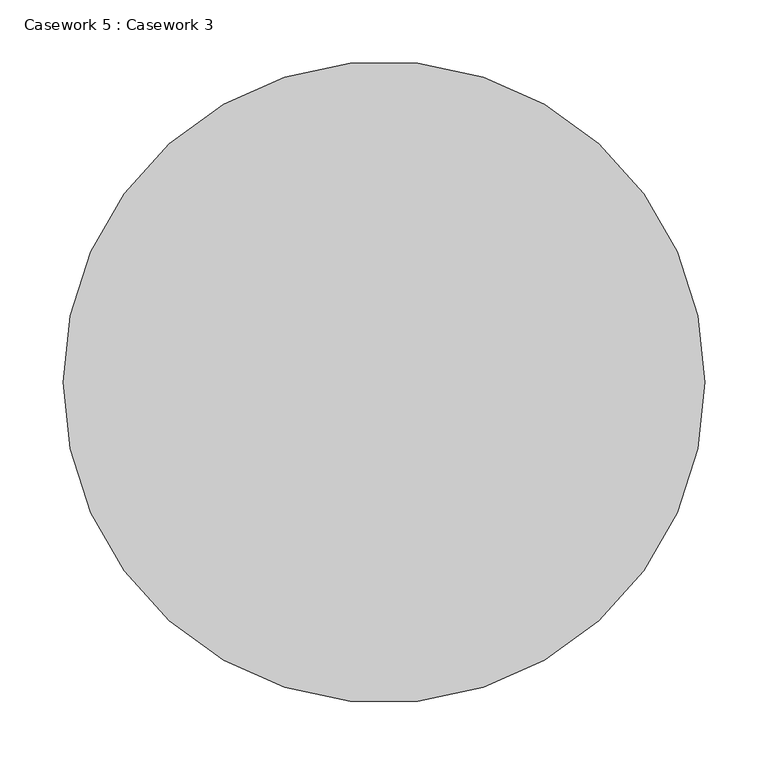
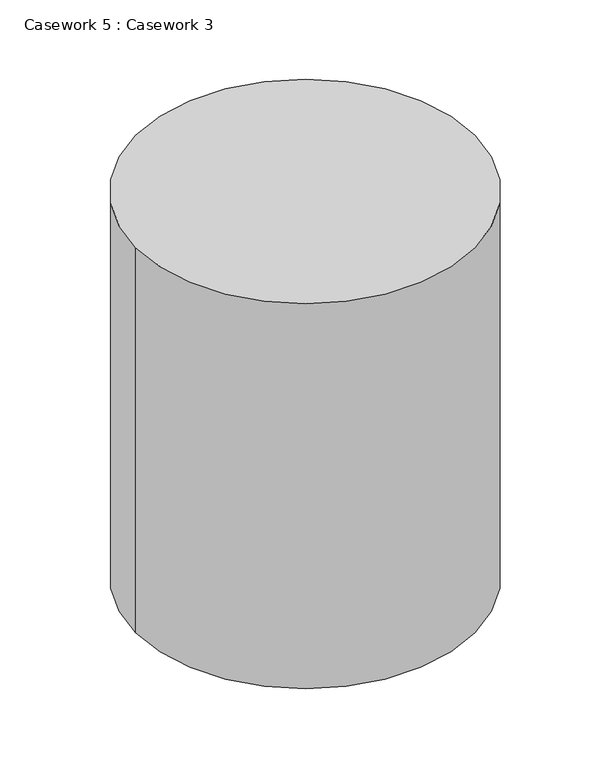
"""IFC4 building model written with IfcOpenShell, lengths in millimetres: furniture geometry, Casework 5 : Casework 3."""

import ifcopenshell
import ifcopenshell.guid

model = None  # the IFC model being written
_history = None  # IfcOwnerHistory: only IFC2X3 demands one
_inside = {}  # id of a spatial element -> (the spatial element, [elements in it])
_under = {}  # id of a project, library or spatial element -> (it, [spatial elements below it])
_declared = {}  # id of a project -> (the project, [libraries it declares])
_typed = {}  # id of a type object -> (the type object, [elements of that type])
_made_of = {}  # id of a material, layer set ... -> (it, [elements and type objects made of it])


def new_model(schema):
    """Start an empty IFC model of exactly this schema.

    Asked for "IFC4X3", IfcOpenShell would pick the latest addendum, in which some entities
    have other attributes; the version numbers below select the first issue.
    IFC2X3 requires an IfcOwnerHistory on every rooted entity: one is made here for all.
    """
    global model, _history
    if schema == "IFC4X3":
        model = ifcopenshell.file(schema_version=(4, 3, 0, 0))
    else:
        model = ifcopenshell.file(schema=schema)
    _inside.clear()
    _under.clear()
    _declared.clear()
    _typed.clear()
    _made_of.clear()
    _history = None
    if model.schema == "IFC2X3":
        org = make("IfcOrganization", Name="unknown")
        user = make(
            "IfcPersonAndOrganization",
            ThePerson=make("IfcPerson", FamilyName="unknown"),
            TheOrganization=org,
        )
        app = make(
            "IfcApplication",
            ApplicationDeveloper=org,
            Version="unknown",
            ApplicationFullName="unknown",
            ApplicationIdentifier="unknown",
        )
        _history = make(
            "IfcOwnerHistory",
            OwningUser=user,
            OwningApplication=app,
            ChangeAction="ADDED",
            CreationDate=0,
        )
    return model


def make(cls, **values):
    """One entity of the class cls with the attributes given. An attribute that is None is left unset."""
    return model.create_entity(
        cls, **{name: value for name, value in values.items() if value is not None}
    )


def rooted(cls, **values):
    """An entity with a GlobalId (a new one), such as an element, a storey or a relation."""
    return make(cls, GlobalId=ifcopenshell.guid.new(), OwnerHistory=_history, **values)


def si_unit(unit_type, name, prefix=None):
    """IfcSIUnit, for example si_unit("LENGTHUNIT", "METRE", prefix="MILLI")."""
    return make("IfcSIUnit", UnitType=unit_type, Prefix=prefix, Name=name)


def assignment(units):
    """IfcUnitAssignment: the units of a project."""
    return None if units is None else make("IfcUnitAssignment", Units=units)


def point(xyz):
    """IfcCartesianPoint."""
    return None if xyz is None else make("IfcCartesianPoint", Coordinates=xyz)


def direction(xyz):
    """IfcDirection."""
    return None if xyz is None else make("IfcDirection", DirectionRatios=xyz)


def frame(location, z_axis=None, x_axis=None):
    """IfcAxis2Placement3D, a coordinate frame: its origin and axes. An axis left out is left unset."""
    return make(
        "IfcAxis2Placement3D",
        Location=point(location),
        Axis=direction(z_axis),
        RefDirection=direction(x_axis),
    )


def frame_2d(location, x_axis=None):
    """IfcAxis2Placement2D, a coordinate frame in the plane: its origin and x axis."""
    return make(
        "IfcAxis2Placement2D", Location=point(location), RefDirection=direction(x_axis)
    )


def origin():
    """The frame at (0, 0, 0) with its axes left unset."""
    return frame((0.0, 0.0, 0.0))


def origin_with_axes():
    """The frame at (0, 0, 0) with the z axis (0, 0, 1) and the x axis (1, 0, 0) written out."""
    return frame((0.0, 0.0, 0.0), z_axis=(0.0, 0.0, 1.0), x_axis=(1.0, 0.0, 0.0))


def place(relative_to, where):
    """IfcLocalPlacement: puts the frame where relative to a parent placement (None: the world)."""
    return make(
        "IfcLocalPlacement", PlacementRelTo=relative_to, RelativePlacement=where
    )


def context(
    kind, dimensions, precision=None, world=None, true_north=None, identifier=None
):
    """IfcGeometricRepresentationContext, for example the 3D "Model" context."""
    return make(
        "IfcGeometricRepresentationContext",
        ContextIdentifier=identifier,
        ContextType=kind,
        CoordinateSpaceDimension=dimensions,
        Precision=precision,
        WorldCoordinateSystem=world,
        TrueNorth=true_north,
    )


def project(units=None, contexts=None):
    """IfcProject with its units and contexts."""
    return rooted(
        "IfcProject",
        Name="project",
        RepresentationContexts=contexts,
        UnitsInContext=assignment(units),
    )


def spatial(cls, under=None, at=None, **own):
    """A site, building, storey or space (cls), placed at a placement, below another one or the project."""
    s = rooted(cls, ObjectPlacement=at, **own)
    if under is not None:
        _under.setdefault(under.id(), (under, []))[1].append(s)
    return s


def circle_curve(where, radius):
    """IfcCircle in the frame where."""
    return make("IfcCircle", Position=where, Radius=radius)


def trimmed(basis, trim1, trim2, sense, master):
    """IfcTrimmedCurve: the piece of a basis curve between two trims."""
    return make(
        "IfcTrimmedCurve",
        BasisCurve=basis,
        Trim1=trim1,
        Trim2=trim2,
        SenseAgreement=sense,
        MasterRepresentation=master,
    )


def segment(curve, same_sense, transition):
    """IfcCompositeCurveSegment."""
    return make(
        "IfcCompositeCurveSegment",
        Transition=transition,
        SameSense=same_sense,
        ParentCurve=curve,
    )


def composite_curve(segments, self_intersect=None):
    """IfcCompositeCurve: segments joined end to end."""
    return make("IfcCompositeCurve", Segments=segments, SelfIntersect=self_intersect)


def outline(outer, holes=None, kind="AREA"):
    """IfcArbitraryClosedProfileDef: a profile drawn as a closed curve; with holes, ...WithVoids."""
    if holes is None:
        return make("IfcArbitraryClosedProfileDef", ProfileType=kind, OuterCurve=outer)
    return make(
        "IfcArbitraryProfileDefWithVoids",
        ProfileType=kind,
        OuterCurve=outer,
        InnerCurves=holes,
    )


def extrude(swept, where, along, depth):
    """IfcExtrudedAreaSolid: the profile swept, set in the frame where, extruded along a direction by depth."""
    return make(
        "IfcExtrudedAreaSolid",
        SweptArea=swept,
        Position=where,
        ExtrudedDirection=direction(along),
        Depth=depth,
    )


def shape(context_of_items, identifier, shape_type, items):
    """IfcShapeRepresentation: the items that make up one representation, for example the "Body"."""
    return make(
        "IfcShapeRepresentation",
        ContextOfItems=context_of_items,
        RepresentationIdentifier=identifier,
        RepresentationType=shape_type,
        Items=items,
    )


def source(mapping_origin, context_of_items, identifier, shape_type, items):
    """IfcRepresentationMap: a shape defined once, which mapped items show again and again."""
    return make(
        "IfcRepresentationMap",
        MappingOrigin=mapping_origin,
        MappedRepresentation=shape(context_of_items, identifier, shape_type, items),
    )


def transform(
    local_origin,
    x_axis=None,
    y_axis=None,
    z_axis=None,
    scale=None,
    scale2=None,
    scale3=None,
    uniform=True,
):
    """IfcCartesianTransformationOperator3D, or its non-uniform kind. x_axis, y_axis, z_axis: its Axis1, 2, 3."""
    if uniform:
        return make(
            "IfcCartesianTransformationOperator3D",
            Axis1=direction(x_axis),
            Axis2=direction(y_axis),
            LocalOrigin=point(local_origin),
            Scale=scale,
            Axis3=direction(z_axis),
        )
    return make(
        "IfcCartesianTransformationOperator3DnonUniform",
        Axis1=direction(x_axis),
        Axis2=direction(y_axis),
        LocalOrigin=point(local_origin),
        Scale=scale,
        Axis3=direction(z_axis),
        Scale2=scale2,
        Scale3=scale3,
    )


def mapped(mapping_source, mapping_target):
    """IfcMappedItem: shows the shape of a source again, moved by a transform."""
    return make(
        "IfcMappedItem", MappingSource=mapping_source, MappingTarget=mapping_target
    )


def made_of(thing, what):
    """Note that an element or type object is made of a material, layer set ...; save() writes the relation."""
    if what is not None:
        _made_of.setdefault(what.id(), (what, []))[1].append(thing)
    return thing


def element(
    cls,
    number,
    at=None,
    inside=None,
    cuts=None,
    type_object=None,
    material=None,
    context=None,
    identifier="Body",
    shape_type=None,
    held_by="IfcProductDefinitionShape",
    body=None,
    shapes=None,
    **own,
):
    """One element of the class cls, such as IfcWall. Its Tag is "e" and its number.

    at: its placement. inside: the storey or other place that contains it. cuts: it is an
    opening in that element (IfcRelVoidsElement). A single representation is given by context,
    identifier, shape_type and body (its items); several are given by shapes. held_by: the class
    of the entity that holds the representations. save() writes the other relations.
    """
    e = rooted(cls, Tag="e%d" % number, ObjectPlacement=at, **own)
    if body is not None:
        shapes = [shape(context, identifier, shape_type, body)]
    if shapes is not None:
        e.Representation = make(held_by, Representations=shapes)
    if inside is not None:
        _inside.setdefault(inside.id(), (inside, []))[1].append(e)
    if cuts is not None:
        rooted(
            "IfcRelVoidsElement", RelatingBuildingElement=cuts, RelatedOpeningElement=e
        )
    if type_object is not None:
        _typed.setdefault(type_object.id(), (type_object, []))[1].append(e)
    return made_of(e, material)


def aggregate(whole, parts):
    """IfcRelAggregates: a whole, such as a stair, and the parts it consists of."""
    return rooted("IfcRelAggregates", RelatingObject=whole, RelatedObjects=parts)


def save(model, path):
    """Write the relations noted so far, then the file.

    IfcRelAggregates (storeys below a building ...), IfcRelContainedInSpatialStructure (elements
    in a storey), IfcRelDefinesByType, IfcRelAssociatesMaterial and IfcRelDeclares: one each for
    every whole, place, type object, material and project.
    """
    for whole, parts in _under.values():
        aggregate(whole, parts)
    for where, things in _inside.values():
        rooted(
            "IfcRelContainedInSpatialStructure",
            RelatedElements=things,
            RelatingStructure=where,
        )
    for kind, things in _typed.values():
        rooted("IfcRelDefinesByType", RelatedObjects=things, RelatingType=kind)
    for what, things in _made_of.values():
        rooted("IfcRelAssociatesMaterial", RelatedObjects=things, RelatingMaterial=what)
    for by, libraries in _declared.values():
        rooted("IfcRelDeclares", RelatingContext=by, RelatedDefinitions=libraries)
    model.write(path)


def casework_5_casework_3_8d9394b4(model_context):
    return source(origin(), model_context, "Body", "SweptSolid", [
        extrude(outline(composite_curve([segment(trimmed(circle_curve(frame_2d((-51057.4433309, 249325.1782081)), 254.0), [point((-51311.4433309, 249325.1782081))], [point((-50803.4433309, 249325.1782081))], False, "CARTESIAN"), True, "CONTINUOUS"), segment(trimmed(circle_curve(frame_2d((-51057.4433309, 249325.1782081)), 254.0), [point((-50803.4433309, 249325.1782081))], [point((-51311.4433309, 249325.1782081))], False, "CARTESIAN"), True, "CONTINUOUS")], self_intersect=False)), origin_with_axes(), (0.0, 0.0, 1.0), 609.6),
    ])


if __name__ == "__main__":
    model = new_model("IFC4")
    model_context = context("Model", 3, world=origin())
    ifc_project = project(units=[si_unit("LENGTHUNIT", "METRE", prefix="MILLI")], contexts=[model_context])
    site = spatial("IfcSite", under=ifc_project)
    building = spatial("IfcBuilding", under=site)
    placement = place(None, origin())
    casework_5_casework_3_shape = casework_5_casework_3_8d9394b4(model_context)
    element("IfcFurniture", 1, ObjectType="Casework 5 : Casework 3", at=placement, inside=building, context=model_context, shape_type="MappedRepresentation", body=[
        mapped(casework_5_casework_3_shape, transform((0.0, 0.0, 0.0), x_axis=(1.0, 0.0, 0.0), y_axis=(0.0, 1.0, 0.0), z_axis=(0.0, 0.0, 1.0))),
    ])
    save(model, "model.ifc")

# Revit data of these elements
# Element 1 (IfcFurniture, "Casework 5 : Casework 3")
#   Materials on its faces: "TRASH"
# Materials
#   "TRASH": class "Generic", colour RGB 187 187 187, transparency 0, Cost = 0
